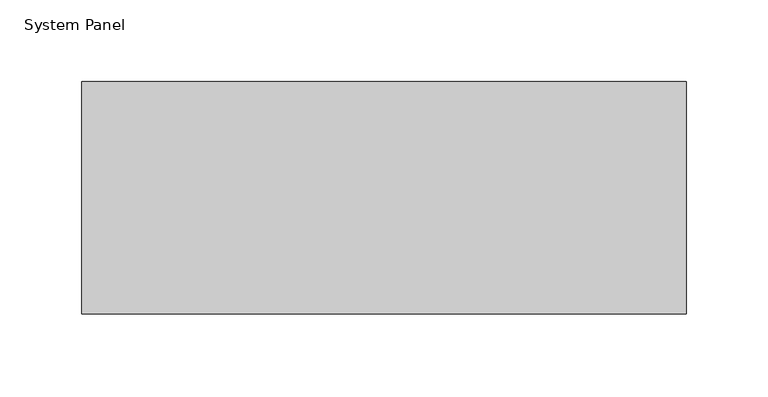
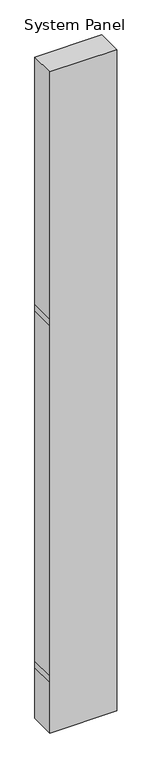
"""IFC4 building model written with IfcOpenShell, lengths in millimetres: plate geometry, System Panel : NLRS_21_CWP_hsb-vulling minerale wol 142 _gen_rsf."""

from ifc_helpers import new_model, si_unit, frame, origin, place, context, project, spatial, polyline, outline, extrude, source, transform, mapped, element, save


def system_panel_efc5a8ab(model_context):
    return source(origin(), model_context, "Body", "SweptSolid", [
        extrude(outline(polyline([(0.0, -184.5), (0.0, 184.5), (295.0, 184.5), (333.0, 184.5), (2371.0, 184.5), (2409.0, 184.5), (3849.0, 184.5), (3849.0, -184.5), (2409.0, -184.5), (2371.0, -184.5), (333.0, -184.5), (295.0, -184.5), (0.0, -184.5)])), frame((0.0, -71.0, 0.0), z_axis=(0.0, 1.0, 0.0), x_axis=(0.0, 0.0, 1.0)), (0.0, 0.0, 1.0), 142.0),
    ])


if __name__ == "__main__":
    model = new_model("IFC4")
    model_context = context("Model", 3, world=origin())
    ifc_project = project(units=[si_unit("LENGTHUNIT", "METRE", prefix="MILLI")], contexts=[model_context])
    site = spatial("IfcSite", under=ifc_project)
    building = spatial("IfcBuilding", under=site)
    placement = place(None, origin())
    system_panel_shape = system_panel_efc5a8ab(model_context)
    element("IfcPlate", 1, ObjectType="System Panel : NLRS_21_CWP_hsb-vulling minerale wol 142 _gen_rsf", at=placement, inside=building, context=model_context, shape_type="MappedRepresentation", body=[
        mapped(system_panel_shape, transform((0.0, 0.0, 0.0), x_axis=(1.0, 0.0, 0.0), y_axis=(0.0, 1.0, 0.0), z_axis=(0.0, 0.0, 1.0))),
    ])
    save(model, "model.ifc")

# Revit data of these elements
# Type "System Panel : NLRS_21_CWP_hsb-vulling minerale wol 142 _gen_rsf"
#   Export Type to IFC As = "IfcWall"
#   Type IfcGUID = "07M7mRoiH1CR8m_RSKIwpC"
#   Assembly Code = "21.23"
# Element 1 (IfcPlate, "System Panel : NLRS_21_CWP_hsb-vulling minerale wol 142 _gen_rsf")
#   Materials on its faces: "NLRS_m1_isolatie minerale wol_gen_rsf"
# Materials
#   "NLRS_m1_isolatie minerale wol_gen_rsf": class "M - Anorganische materialen", colour RGB 200 200 140, transparency 0, Keynote = "m1", Manufacturer = "Revit Standards Foundation", URL = "www.revitstandards.org", Description = "isolatie minerale wol", Cost = 0
